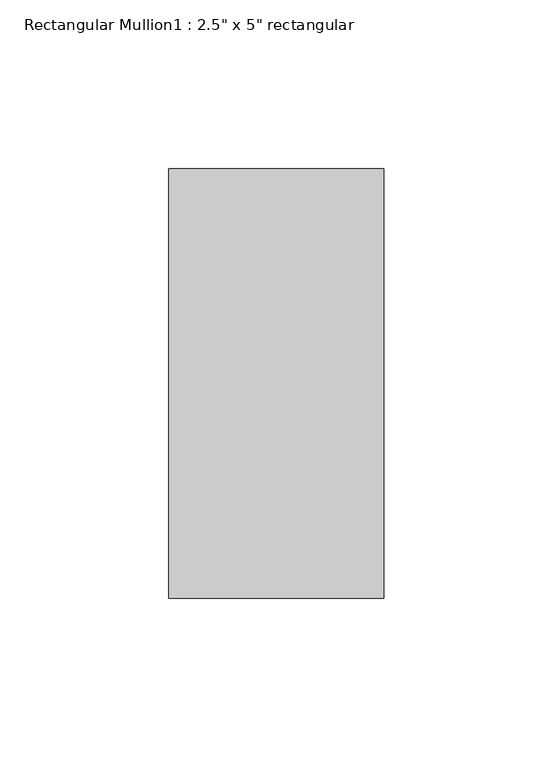
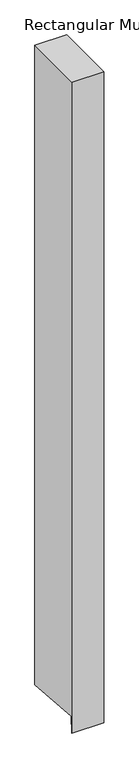
"""IFC4 building model written with IfcOpenShell, lengths in millimetres: member geometry."""

from ifc_helpers import new_model, si_unit, frame, origin, place, context, project, spatial, polyline, outline, extrude, source, transform, mapped, element, save


def member_2f5ef470(model_context):
    return source(origin(), model_context, "Body", "SweptSolid", [
        extrude(outline(polyline([(-63.5, 0.0), (63.5, 0.0), (63.5, -1344.0500431), (-60.9736199, -1334.8041085), (-63.5, -1368.815562), (-63.5, 0.0)])), frame((-63.5, 0.0, 0.0), z_axis=(1.0, 0.0, 0.0), x_axis=(0.0, 1.0, 0.0)), (0.0, 0.0, 1.0), 63.5),
    ])


if __name__ == "__main__":
    model = new_model("IFC4")
    model_context = context("Model", 3, world=origin())
    ifc_project = project(units=[si_unit("LENGTHUNIT", "METRE", prefix="MILLI")], contexts=[model_context])
    site = spatial("IfcSite", under=ifc_project)
    building = spatial("IfcBuilding", under=site)
    placement = place(None, origin())
    member_shape = member_2f5ef470(model_context)
    element("IfcMember", 1, ObjectType="Rectangular Mullion1 : 2.5\" x 5\" rectangular", at=placement, inside=building, context=model_context, shape_type="MappedRepresentation", body=[
        mapped(member_shape, transform((0.0, 0.0, 0.0), x_axis=(1.0, 0.0, 0.0), y_axis=(0.0, 1.0, 0.0), z_axis=(0.0, 0.0, 1.0))),
    ])
    save(model, "model.ifc")

# Revit data of these elements
# Type "Rectangular Mullion1 : 2.5\" x 5\" rectangular"
#   built-in parameter 1007304 = 0.416667 (stored number, unit not read)
#   built-in parameter 1007301 = 0.104167 (stored number, unit not read)
#   built-in parameter 1007300 = 0.104167 (stored number, unit not read)
# Element 1 (IfcMember, "Rectangular Mullion1 : 2.5\" x 5\" rectangular")
#   Materials on its faces: "support-frame"
# Materials
#   "support-frame": class "Unassigned", colour RGB 233 233 233, transparency 0, Cost = 0
